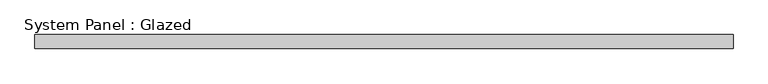
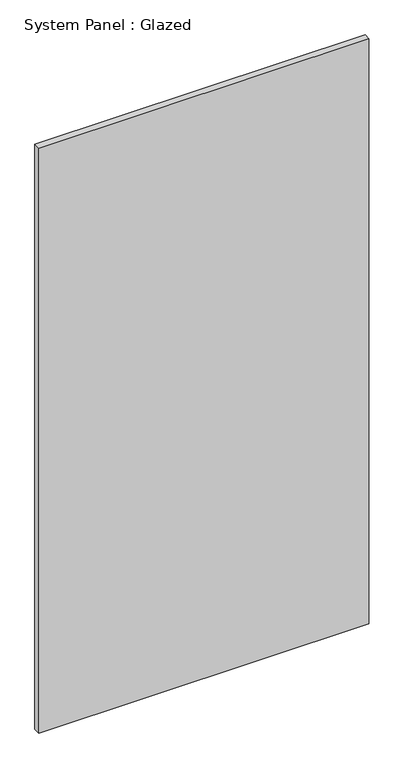
"""IFC4 building model written with IfcOpenShell, lengths in millimetres: plate geometry, System Panel : Glazed."""

from ifc_helpers import new_model, si_unit, origin, origin_with_axes, place, context, project, spatial, polyline, outline, extrude, source, transform, mapped, element, save


def system_panel_glazed_6c662813(model_context):
    return source(origin(), model_context, "Body", "SweptSolid", [
        extrude(outline(polyline([(620.5541356, 24.5), (-620.5541356, 24.5), (-620.5541356, 49.5), (620.5541356, 49.5), (620.5541356, 24.5)])), origin_with_axes(), (0.0, 0.0, 1.0), 2325.0),
    ])


if __name__ == "__main__":
    model = new_model("IFC4")
    model_context = context("Model", 3, world=origin())
    ifc_project = project(units=[si_unit("LENGTHUNIT", "METRE", prefix="MILLI")], contexts=[model_context])
    site = spatial("IfcSite", under=ifc_project)
    building = spatial("IfcBuilding", under=site)
    placement = place(None, origin())
    system_panel_glazed_shape = system_panel_glazed_6c662813(model_context)
    element("IfcPlate", 1, ObjectType="System Panel : Glazed", at=placement, inside=building, context=model_context, shape_type="MappedRepresentation", body=[
        mapped(system_panel_glazed_shape, transform((0.0, 0.0, 0.0), x_axis=(1.0, 0.0, 0.0), y_axis=(0.0, 1.0, 0.0), z_axis=(0.0, 0.0, 1.0))),
    ])
    save(model, "model.ifc")

# Revit data of these elements
# Type "System Panel : Glazed"
#   Construction Type Id = "GSP4R"
#   Analytic Construction = "1/8 in Pilkington single glazing"
#   Visual Light Transmittance = 0.9
#   Solar Heat Gain Coefficient = 0.86
#   Heat Transfer Coefficient (U) = 6.7069 W/(m²·K)
#   Define Thermal Properties by = 1
# Element 1 (IfcPlate, "System Panel : Glazed")
#   Materials on its faces: "Glass"
# Materials
#   "Glass": class "Glass", colour RGB 0 128 192, transparency 0.9, Description = "Soda Lime Glass", Cost = 0
